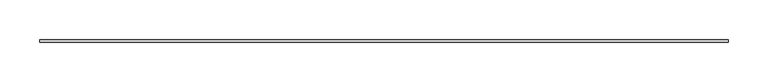
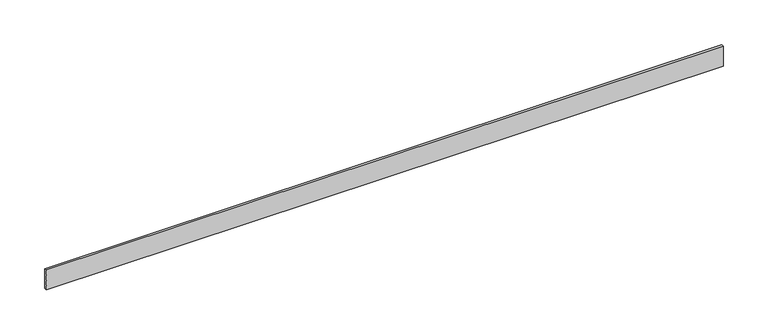
"""IFC4 building model written with IfcOpenShell, lengths in millimetres: proxy geometry, Generic Models 3:Generic Models 1:3:Generic Models 1:3 : Generic Models 3:Generic Models 1:300625:336034:Generic Models 1:3:Generic Models 1:3 : Generic Models 3:Generic Models 1:300625:336034 : Generic Models 3:Generic Models 1:3:Generic Models 1:3 : Generic Models 3:Generic Models 1:300625:336034:5 : Generic Models 3:Generic Models 1:3:Generic Models 1:3 : Generic Models 3:Generic Models 1:300625:336034:Generic Models 1:3:Generic Models 1:3 : Generic Models 3:Generic Models 1:300625:336034 : Generic Models 3:Generic Models 1:3:Generic Models 1:3 : Generic Models 3:Generic Models 1:300625:336034:301191."""

from ifc_helpers import new_model, si_unit, frame, origin, place, context, project, spatial, polyline, outline, extrude, source, transform, mapped, element, save


def generic_models_ada58c09(model_context):
    return source(origin(), model_context, "Body", "SweptSolid", [
        extrude(outline(polyline([(570395.4867239, -579000.6913841), (570395.4867239, -579003.8663841), (569527.1242239, -579003.8663841), (569527.1242239, -579000.6913841), (570395.4867239, -579000.6913841)])), frame((0.0, 0.0, 2446.5359375), z_axis=(0.0, 0.0, 1.0), x_axis=(1.0, 0.0, 0.0)), (0.0, 0.0, 1.0), 26.9875),
    ])


if __name__ == "__main__":
    model = new_model("IFC4")
    model_context = context("Model", 3, world=origin())
    ifc_project = project(units=[si_unit("LENGTHUNIT", "METRE", prefix="MILLI")], contexts=[model_context])
    site = spatial("IfcSite", under=ifc_project)
    building = spatial("IfcBuilding", under=site)
    placement = place(None, origin())
    generic_models_shape = generic_models_ada58c09(model_context)
    element("IfcBuildingElementProxy", 1, Name="Generic Models 3:Generic Models 1:3:Generic Models 1:3 : Generic Models 3:Generic Models 1:300625:336034:Generic Models 1:3:Generic Models 1:3 : Generic Models 3:Generic Models 1:300625:336034 : Generic Models 3:Generic Models 1:3:Generic Models 1:3 : Generic Models 3:Generic Models 1:300625:336034:5 : Generic Models 3:Generic Models 1:3:Generic Models 1:3 : Generic Models 3:Generic Models 1:300625:336034:Generic Models 1:3:Generic Models 1:3 : Generic Models 3:Generic Models 1:300625:336034 : Generic Models 3:Generic Models 1:3:Generic Models 1:3 : Generic Models 3:Generic Models 1:300625:336034:301191", ObjectType="Generic Models 3:Generic Models 1:3:Generic Models 1:3 : Generic Models 3:Generic Models 1:300625:336034:Generic Models 1:3:Generic Models 1:3 : Generic Models 3:Generic Models 1:300625:336034 : Generic Models 3:Generic Models 1:3:Generic Models 1:3 : Generic Models 3:Generic Models 1:300625:336034:5 : Generic Models 3:Generic Models 1:3:Generic Models 1:3 : Generic Models 3:Generic Models 1:300625:336034:Generic Models 1:3:Generic Models 1:3 : Generic Models 3:Generic Models 1:300625:336034 : Generic Models 3:Generic Models 1:3:Generic Models 1:3 : Generic Models 3:Generic Models 1:300625:336034:301191", at=placement, inside=building, context=model_context, shape_type="MappedRepresentation", body=[
        mapped(generic_models_shape, transform((0.0, 0.0, 0.0), x_axis=(1.0, 0.0, 0.0), y_axis=(0.0, 1.0, 0.0), z_axis=(0.0, 0.0, 1.0))),
    ])
    save(model, "model.ifc")

# Revit data of these elements
# Type "Generic Models 3:Generic Models 1:3:Generic Models 1:3 : Generic Models 3:Generic Models 1:300625:336034:Generic Models 1:3:Generic Models 1:3 : Generic Models 3:Generic Models 1:300625:336034 : Generic Models 3:Generic Models 1:3:Generic Models 1:3 : Generic Models 3:Generic Models 1:300625:336034:5 : Generic Models 3:Generic Models 1:3:Generic Models 1:3 : Generic Models 3:Generic Models 1:300625:336034:Generic Models 1:3:Generic Models 1:3 : Generic Models 3:Generic Models 1:300625:336034 : Generic Models 3:Generic Models 1:3:Generic Models 1:3 : Generic Models 3:Generic Models 1:300625:336034:301191"
#   NameOverride = "Generic Models 3:Generic Models 1:3:Generic Models 1:3 : Generic Models 3:Generic Models 1:300625:336034:Generic Models 1:3:Generic Models 1:3 : Generic Models 3:Generic Models 1:300625:336034 : Generic Models 3:Generic Models 1:3:Generic Models 1:3 : Generic Models 3:Generic Models 1:300625:336034:301191"
#   ObjectTypeOverride = "Generic Models 1:3:Generic Models 1:3 : Generic Models 3:Generic Models 1:300625:336034 : Generic Models 3:Generic Models 1:3:Generic Models 1:3 : Generic Models 3:Generic Models 1:300625:336034"
#   Reference = "Generic Models 1"
#   Tag = "301191"
# Element 1 (IfcBuildingElementProxy, "Generic Models 3:Generic Models 1:3:Generic Models 1:3 : Generic Models 3:Generic Models 1:300625:336034:Generic Models 1:3:Generic Models 1:3 : Generic Models 3:Generic Models 1:300625:336034 : Generic Models 3:Generic Models 1:3:Generic Models 1:3 : Generic Models 3:Generic Models 1:300625:336034:5 : Generic Models 3:Generic Models 1:3:Generic Models 1:3 : Generic Models 3:Generic Models 1:300625:336034:Generic Models 1:3:Generic Models 1:3 : Generic Models 3:Generic Models 1:300625:336034 : Generic Models 3:Generic Models 1:3:Generic Models 1:3 : Generic Models 3:Generic Models 1:300625:336034:301191")
#   Materials on its faces: "COMPRESSIBE THERMAL GASKET SANDWICHED BETWEEN METAL COMPONENTS"
# Materials
#   "COMPRESSIBE THERMAL GASKET SANDWICHED BETWEEN METAL COMPONENTS": class "Unassigned", colour RGB 58 208 21, transparency 0, Cost = 0
